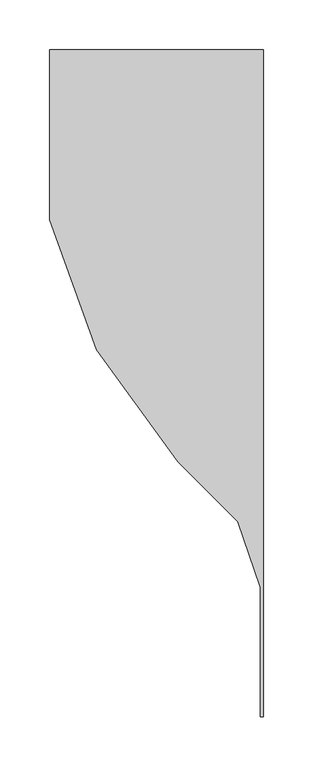
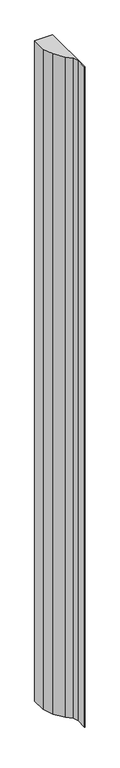
"""IFC4 building model written with IfcOpenShell, lengths in millimetres: proxy geometry, Generic Models 2:Generic Models 2:310765:Generic Models 2:310765 : Generic Models 2:Generic Models 2:310765:72 : Generic Models 2:Generic Models 2:310765:Generic Models 2:310765 : Generic Models 2:Generic Models 2:310765:300385."""

import ifcopenshell
import ifcopenshell.guid

model = None  # the IFC model being written
_history = None  # IfcOwnerHistory: only IFC2X3 demands one
_inside = {}  # id of a spatial element -> (the spatial element, [elements in it])
_under = {}  # id of a project, library or spatial element -> (it, [spatial elements below it])
_declared = {}  # id of a project -> (the project, [libraries it declares])
_typed = {}  # id of a type object -> (the type object, [elements of that type])
_made_of = {}  # id of a material, layer set ... -> (it, [elements and type objects made of it])


def new_model(schema):
    """Start an empty IFC model of exactly this schema.

    Asked for "IFC4X3", IfcOpenShell would pick the latest addendum, in which some entities
    have other attributes; the version numbers below select the first issue.
    IFC2X3 requires an IfcOwnerHistory on every rooted entity: one is made here for all.
    """
    global model, _history
    if schema == "IFC4X3":
        model = ifcopenshell.file(schema_version=(4, 3, 0, 0))
    else:
        model = ifcopenshell.file(schema=schema)
    _inside.clear()
    _under.clear()
    _declared.clear()
    _typed.clear()
    _made_of.clear()
    _history = None
    if model.schema == "IFC2X3":
        org = make("IfcOrganization", Name="unknown")
        user = make(
            "IfcPersonAndOrganization",
            ThePerson=make("IfcPerson", FamilyName="unknown"),
            TheOrganization=org,
        )
        app = make(
            "IfcApplication",
            ApplicationDeveloper=org,
            Version="unknown",
            ApplicationFullName="unknown",
            ApplicationIdentifier="unknown",
        )
        _history = make(
            "IfcOwnerHistory",
            OwningUser=user,
            OwningApplication=app,
            ChangeAction="ADDED",
            CreationDate=0,
        )
    return model


def make(cls, **values):
    """One entity of the class cls with the attributes given. An attribute that is None is left unset."""
    return model.create_entity(
        cls, **{name: value for name, value in values.items() if value is not None}
    )


def rooted(cls, **values):
    """An entity with a GlobalId (a new one), such as an element, a storey or a relation."""
    return make(cls, GlobalId=ifcopenshell.guid.new(), OwnerHistory=_history, **values)


def si_unit(unit_type, name, prefix=None):
    """IfcSIUnit, for example si_unit("LENGTHUNIT", "METRE", prefix="MILLI")."""
    return make("IfcSIUnit", UnitType=unit_type, Prefix=prefix, Name=name)


def assignment(units):
    """IfcUnitAssignment: the units of a project."""
    return None if units is None else make("IfcUnitAssignment", Units=units)


def point(xyz):
    """IfcCartesianPoint."""
    return None if xyz is None else make("IfcCartesianPoint", Coordinates=xyz)


def direction(xyz):
    """IfcDirection."""
    return None if xyz is None else make("IfcDirection", DirectionRatios=xyz)


def frame(location, z_axis=None, x_axis=None):
    """IfcAxis2Placement3D, a coordinate frame: its origin and axes. An axis left out is left unset."""
    return make(
        "IfcAxis2Placement3D",
        Location=point(location),
        Axis=direction(z_axis),
        RefDirection=direction(x_axis),
    )


def origin():
    """The frame at (0, 0, 0) with its axes left unset."""
    return frame((0.0, 0.0, 0.0))


def origin_with_axes():
    """The frame at (0, 0, 0) with the z axis (0, 0, 1) and the x axis (1, 0, 0) written out."""
    return frame((0.0, 0.0, 0.0), z_axis=(0.0, 0.0, 1.0), x_axis=(1.0, 0.0, 0.0))


def place(relative_to, where):
    """IfcLocalPlacement: puts the frame where relative to a parent placement (None: the world)."""
    return make(
        "IfcLocalPlacement", PlacementRelTo=relative_to, RelativePlacement=where
    )


def context(
    kind, dimensions, precision=None, world=None, true_north=None, identifier=None
):
    """IfcGeometricRepresentationContext, for example the 3D "Model" context."""
    return make(
        "IfcGeometricRepresentationContext",
        ContextIdentifier=identifier,
        ContextType=kind,
        CoordinateSpaceDimension=dimensions,
        Precision=precision,
        WorldCoordinateSystem=world,
        TrueNorth=true_north,
    )


def project(units=None, contexts=None):
    """IfcProject with its units and contexts."""
    return rooted(
        "IfcProject",
        Name="project",
        RepresentationContexts=contexts,
        UnitsInContext=assignment(units),
    )


def spatial(cls, under=None, at=None, **own):
    """A site, building, storey or space (cls), placed at a placement, below another one or the project."""
    s = rooted(cls, ObjectPlacement=at, **own)
    if under is not None:
        _under.setdefault(under.id(), (under, []))[1].append(s)
    return s


def polyline(points):
    """IfcPolyline through the points."""
    return make("IfcPolyline", Points=[point(p) for p in points])


def outline(outer, holes=None, kind="AREA"):
    """IfcArbitraryClosedProfileDef: a profile drawn as a closed curve; with holes, ...WithVoids."""
    if holes is None:
        return make("IfcArbitraryClosedProfileDef", ProfileType=kind, OuterCurve=outer)
    return make(
        "IfcArbitraryProfileDefWithVoids",
        ProfileType=kind,
        OuterCurve=outer,
        InnerCurves=holes,
    )


def extrude(swept, where, along, depth):
    """IfcExtrudedAreaSolid: the profile swept, set in the frame where, extruded along a direction by depth."""
    return make(
        "IfcExtrudedAreaSolid",
        SweptArea=swept,
        Position=where,
        ExtrudedDirection=direction(along),
        Depth=depth,
    )


def shape(context_of_items, identifier, shape_type, items):
    """IfcShapeRepresentation: the items that make up one representation, for example the "Body"."""
    return make(
        "IfcShapeRepresentation",
        ContextOfItems=context_of_items,
        RepresentationIdentifier=identifier,
        RepresentationType=shape_type,
        Items=items,
    )


def source(mapping_origin, context_of_items, identifier, shape_type, items):
    """IfcRepresentationMap: a shape defined once, which mapped items show again and again."""
    return make(
        "IfcRepresentationMap",
        MappingOrigin=mapping_origin,
        MappedRepresentation=shape(context_of_items, identifier, shape_type, items),
    )


def transform(
    local_origin,
    x_axis=None,
    y_axis=None,
    z_axis=None,
    scale=None,
    scale2=None,
    scale3=None,
    uniform=True,
):
    """IfcCartesianTransformationOperator3D, or its non-uniform kind. x_axis, y_axis, z_axis: its Axis1, 2, 3."""
    if uniform:
        return make(
            "IfcCartesianTransformationOperator3D",
            Axis1=direction(x_axis),
            Axis2=direction(y_axis),
            LocalOrigin=point(local_origin),
            Scale=scale,
            Axis3=direction(z_axis),
        )
    return make(
        "IfcCartesianTransformationOperator3DnonUniform",
        Axis1=direction(x_axis),
        Axis2=direction(y_axis),
        LocalOrigin=point(local_origin),
        Scale=scale,
        Axis3=direction(z_axis),
        Scale2=scale2,
        Scale3=scale3,
    )


def mapped(mapping_source, mapping_target):
    """IfcMappedItem: shows the shape of a source again, moved by a transform."""
    return make(
        "IfcMappedItem", MappingSource=mapping_source, MappingTarget=mapping_target
    )


def made_of(thing, what):
    """Note that an element or type object is made of a material, layer set ...; save() writes the relation."""
    if what is not None:
        _made_of.setdefault(what.id(), (what, []))[1].append(thing)
    return thing


def element(
    cls,
    number,
    at=None,
    inside=None,
    cuts=None,
    type_object=None,
    material=None,
    context=None,
    identifier="Body",
    shape_type=None,
    held_by="IfcProductDefinitionShape",
    body=None,
    shapes=None,
    **own,
):
    """One element of the class cls, such as IfcWall. Its Tag is "e" and its number.

    at: its placement. inside: the storey or other place that contains it. cuts: it is an
    opening in that element (IfcRelVoidsElement). A single representation is given by context,
    identifier, shape_type and body (its items); several are given by shapes. held_by: the class
    of the entity that holds the representations. save() writes the other relations.
    """
    e = rooted(cls, Tag="e%d" % number, ObjectPlacement=at, **own)
    if body is not None:
        shapes = [shape(context, identifier, shape_type, body)]
    if shapes is not None:
        e.Representation = make(held_by, Representations=shapes)
    if inside is not None:
        _inside.setdefault(inside.id(), (inside, []))[1].append(e)
    if cuts is not None:
        rooted(
            "IfcRelVoidsElement", RelatingBuildingElement=cuts, RelatedOpeningElement=e
        )
    if type_object is not None:
        _typed.setdefault(type_object.id(), (type_object, []))[1].append(e)
    return made_of(e, material)


def aggregate(whole, parts):
    """IfcRelAggregates: a whole, such as a stair, and the parts it consists of."""
    return rooted("IfcRelAggregates", RelatingObject=whole, RelatedObjects=parts)


def save(model, path):
    """Write the relations noted so far, then the file.

    IfcRelAggregates (storeys below a building ...), IfcRelContainedInSpatialStructure (elements
    in a storey), IfcRelDefinesByType, IfcRelAssociatesMaterial and IfcRelDeclares: one each for
    every whole, place, type object, material and project.
    """
    for whole, parts in _under.values():
        aggregate(whole, parts)
    for where, things in _inside.values():
        rooted(
            "IfcRelContainedInSpatialStructure",
            RelatedElements=things,
            RelatingStructure=where,
        )
    for kind, things in _typed.values():
        rooted("IfcRelDefinesByType", RelatedObjects=things, RelatingType=kind)
    for what, things in _made_of.values():
        rooted("IfcRelAssociatesMaterial", RelatedObjects=things, RelatingMaterial=what)
    for by, libraries in _declared.values():
        rooted("IfcRelDeclares", RelatingContext=by, RelatedDefinitions=libraries)
    model.write(path)


def generic_models_1fc4fe35(model_context):
    return source(origin(), model_context, "Body", "SweptSolid", [
        extrude(outline(polyline([(757365.9431628, -567542.1163841), (757581.8431628, -567542.1163841), (757581.8431628, -568215.2163841), (757579.1204, -568215.2163841), (757579.1204, -568084.3267825), (757556.4431628, -568018.4673036), (757495.8369766, -567957.8611173), (757413.7233768, -567844.8414432), (757365.9431628, -567713.5663841), (757365.9431628, -567542.1163841)])), origin_with_axes(), (0.0, 0.0, 1.0), 8407.9758546),
    ])


if __name__ == "__main__":
    model = new_model("IFC4")
    model_context = context("Model", 3, world=origin())
    ifc_project = project(units=[si_unit("LENGTHUNIT", "METRE", prefix="MILLI")], contexts=[model_context])
    site = spatial("IfcSite", under=ifc_project)
    building = spatial("IfcBuilding", under=site)
    placement = place(None, origin())
    generic_models_shape = generic_models_1fc4fe35(model_context)
    element("IfcBuildingElementProxy", 1, Name="Generic Models 2:Generic Models 2:310765:Generic Models 2:310765 : Generic Models 2:Generic Models 2:310765:72 : Generic Models 2:Generic Models 2:310765:Generic Models 2:310765 : Generic Models 2:Generic Models 2:310765:300385", ObjectType="Generic Models 2:Generic Models 2:310765:Generic Models 2:310765 : Generic Models 2:Generic Models 2:310765:72 : Generic Models 2:Generic Models 2:310765:Generic Models 2:310765 : Generic Models 2:Generic Models 2:310765:300385", at=placement, inside=building, context=model_context, shape_type="MappedRepresentation", body=[
        mapped(generic_models_shape, transform((0.0, 0.0, 0.0), x_axis=(1.0, 0.0, 0.0), y_axis=(0.0, 1.0, 0.0), z_axis=(0.0, 0.0, 1.0))),
    ])
    save(model, "model.ifc")

# Revit data of these elements
# Type "Generic Models 2:Generic Models 2:310765:Generic Models 2:310765 : Generic Models 2:Generic Models 2:310765:72 : Generic Models 2:Generic Models 2:310765:Generic Models 2:310765 : Generic Models 2:Generic Models 2:310765:300385"
#   NameOverride = "Generic Models 2:Generic Models 2:310765:Generic Models 2:310765 : Generic Models 2:Generic Models 2:310765:300385"
#   ObjectTypeOverride = "Generic Models 2:310765 : Generic Models 2:Generic Models 2:310765"
#   Reference = "Generic Models 2"
#   Tag = "300385"
# Element 1 (IfcBuildingElementProxy, "Generic Models 2:Generic Models 2:310765:Generic Models 2:310765 : Generic Models 2:Generic Models 2:310765:72 : Generic Models 2:Generic Models 2:310765:Generic Models 2:310765 : Generic Models 2:Generic Models 2:310765:300385")
#   Materials on its faces: "CLASS A FIBERGLASS INSULATION WITH DURABLE VAPOR BARRIER (WHITE) LINE"
# Materials
#   "CLASS A FIBERGLASS INSULATION WITH DURABLE VAPOR BARRIER (WHITE) LINE": class "Unassigned", colour RGB 187 139 199, transparency 0, Cost = 0
